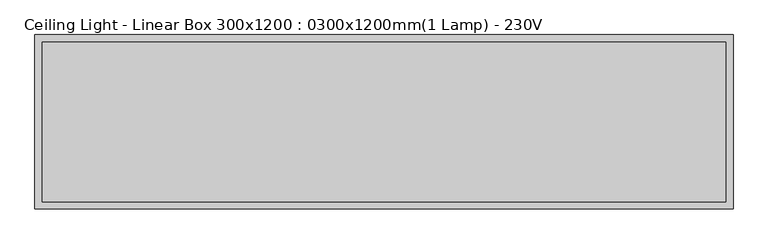
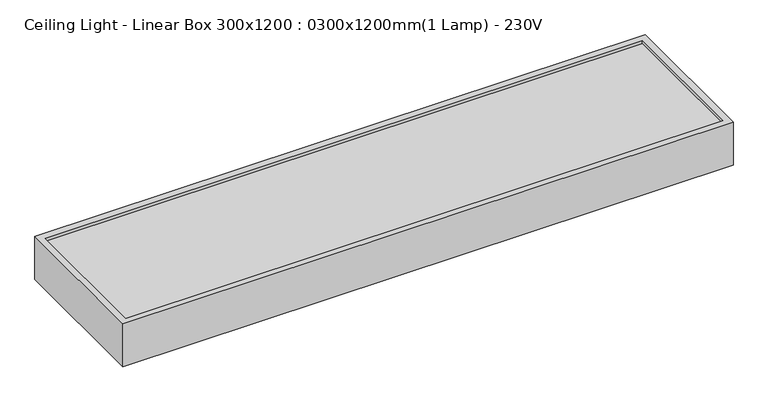
"""IFC4 building model written with IfcOpenShell, lengths in millimetres: light fixture geometry, Ceiling Light - Linear Box 300x1200 : 0300x1200mm(1 Lamp) - 230V."""

from ifc_helpers import new_model, si_unit, frame, origin, origin_with_axes, place, context, project, spatial, polyline, outline, extrude, source, transform, mapped, element, save


def ceiling_light_linear_box_300x1200_0300x1200mm_1_lamp_230v_9b76a469(model_context):
    return source(origin(), model_context, "Body", "SweptSolid", [
        extrude(outline(polyline([(587.3, -12.7), (587.3, -287.3), (-587.3, -287.3), (-587.3, -12.7), (587.3, -12.7)])), frame((0.0, 0.0, 76.2), z_axis=(0.0, 0.0, 1.0), x_axis=(1.0, 0.0, 0.0)), (0.0, 0.0, 1.0), 6.35),
        extrude(outline(polyline([(600.0, 0.0), (600.0, -300.0), (-600.0, -300.0), (-600.0, 0.0), (600.0, 0.0)]), holes=[polyline([(587.3, -12.7), (-587.3, -12.7), (-587.3, -287.3), (587.3, -287.3), (587.3, -12.7)])]), origin_with_axes(), (0.0, 0.0, 1.0), 88.9),
    ])


if __name__ == "__main__":
    model = new_model("IFC4")
    model_context = context("Model", 3, world=origin())
    ifc_project = project(units=[si_unit("LENGTHUNIT", "METRE", prefix="MILLI")], contexts=[model_context])
    site = spatial("IfcSite", under=ifc_project)
    building = spatial("IfcBuilding", under=site)
    placement = place(None, origin())
    ceiling_light_linear_box_300x1200_0300x1200mm_1_lamp_230v_shape = ceiling_light_linear_box_300x1200_0300x1200mm_1_lamp_230v_9b76a469(model_context)
    element("IfcLightFixture", 1, ObjectType="Ceiling Light - Linear Box 300x1200 : 0300x1200mm(1 Lamp) - 230V", at=placement, inside=building, context=model_context, shape_type="MappedRepresentation", body=[
        mapped(ceiling_light_linear_box_300x1200_0300x1200mm_1_lamp_230v_shape, transform((0.0, 0.0, 0.0), x_axis=(1.0, 0.0, 0.0), y_axis=(0.0, 1.0, 0.0), z_axis=(0.0, 0.0, 1.0))),
    ])
    save(model, "model.ifc")

# Revit data of these elements
# Type "Ceiling Light - Linear Box 300x1200 : 0300x1200mm(1 Lamp) - 230V"
#   Type Mark = "Ceiling Light - Linear Box 300x1200"
#   Classification.OmniClass.23.Number = "23-35 47 11"
#   Classification.OmniClass.23.Description = "Lighting Fixtures"
#   COBie.Type.CreatedBy = "info@mma.ie"
#   COBie.Type.CreatedOn = "2017-07-25T10:15:16"
#   COBie.Type.Name = "Ceiling Light - Linear Box 300x1200"
#   COBie.Type.Category = "23-35 47 11 : Lighting Fixtures"
#   COBie.Type.Description = "Ceiling Light - Linear Box 300x1200_0300x1200mm(1 Lamp) - 230V"
#   COBie.Type.AssetType = "Fixed"
#   COBie.Type.Manufacturer = ""
#   COBie.Type.ModelNumber = ""
#   Photometric Web File = "1x41T12.ies"
#   Lamp = "T-12"
#   Keynote = "26 51 13.A"
#   Assembly Code = "D5020210"
#   COBie.Type.ReplacementCost = 0
#   Width 1 = 150 mm
#   Wattage = 40 W
#   built-in parameter 1150110 = 1 (stored number, unit not read)
#   built-in parameter 1114217 = 0.88 (stored number, unit not read)
#   built-in parameter 1150109 = 1 (stored number, unit not read)
#   built-in parameter 1150113 = 1 (stored number, unit not read)
#   Tilt Angle = -90.00°
#   Lumens = 3150 lm
#   built-in parameter 1150115 = 1 (stored number, unit not read)
#   built-in parameter 1150105 = 250.669 (stored number, unit not read)
#   Length1 = 600 mm
#   built-in parameter 1150112 = 1 (stored number, unit not read)
#   built-in parameter 1150114 = 1 (stored number, unit not read)
#   built-in parameter 1150107 = 4230 (stored number, unit not read)
#   built-in parameter 1150106 = 2.50669 (stored number, unit not read)
#   Emit from Rectangle Width = 274 mm
#   Emit from Rectangle Length = 1174 mm
#   built-in parameter 1150104 = 7.31611 (stored number, unit not read)
#   Default Elevation = 1200 mm
#   C.L. Width = 300 mm
#   C.L. Length = 1200 mm
#   C.L. Depth = 88.9 mm
#   Ballast Voltage = 230 V
#   built-in parameter 1114218 = 0.88 (stored number, unit not read)
#   built-in parameter 1150133 = 10 (stored number, unit not read)
#   Apparent Load = 40 VA
#   COBie.Type = yes
#   built-in parameter 1150134 = 8
#   built-in parameter 1150137 = 1
#   Color Filter = 16777215
#   built-in parameter 1140040 [instance default] = 1
#   Ballast Number of Poles = 1
#   Load Classification = Lighting - Dwelling Unit
#   Light Box Material = Metal - Paint Finish - Ivory, Glossy
#   Diffuser Material = Glass - White, High Luminance
#   BLACK = Phase - Demo
#   Emit Shape Visible in Rendering = no
#   Dimming Lamp Color Temperature Shift = (empty or 0)
# Element 1 (IfcLightFixture, "Ceiling Light - Linear Box 300x1200 : 0300x1200mm(1 Lamp) - 230V")
#   Materials on its faces: "Phase - Demo", "Glass - White, High Luminance"
# Materials
#   "Metal - Paint Finish - Ivory, Glossy": class "Paint", colour RGB 247 247 239, transparency 0, Comments = "Rendering appearance not upgraded "
#   "Glass - White, High Luminance": class "Glass", colour RGB 249 250 249, transparency 0.8
#   "Phase - Demo": class "System", colour RGB 255 0 0, transparency 0.4
